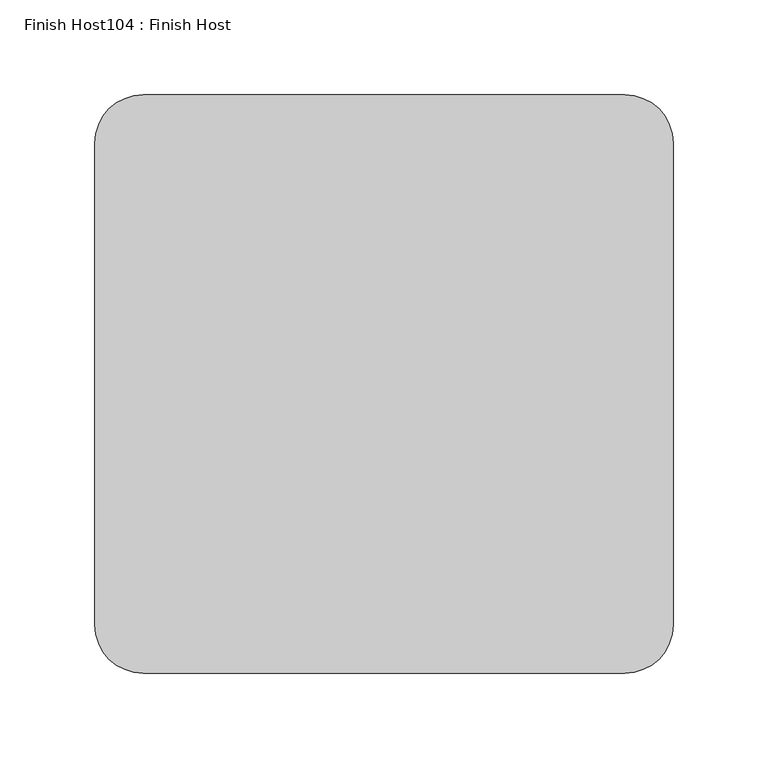
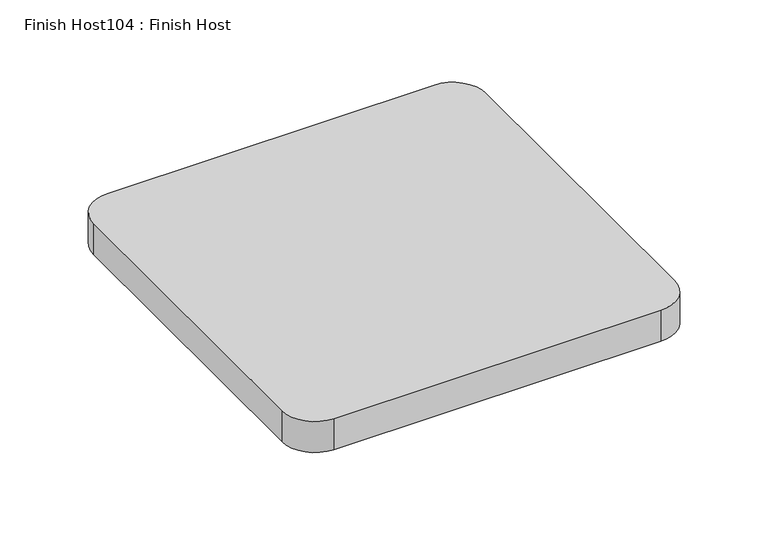
"""IFC4 building model written with IfcOpenShell, lengths in millimetres: proxy geometry, Finish Host104 : Finish Host."""

from ifc_helpers import new_model, si_unit, point, frame_2d, origin, origin_with_axes, place, context, project, spatial, polyline, circle_curve, trimmed, segment, composite_curve, outline, extrude, source, transform, mapped, element, save


def finish_host104_finish_host_b2d7b205(model_context):
    return source(origin(), model_context, "Body", "SweptSolid", [
        extrude(outline(composite_curve([segment(polyline([(701.4157184, 4229.4760864), (701.4157184, 4483.4760864)]), True, "CONTINUOUS"), segment(trimmed(circle_curve(frame_2d((726.8157184, 4483.4760864)), 25.4), [point((701.4157184, 4483.4760864))], [point((726.8157184, 4508.8760864))], False, "CARTESIAN"), True, "CONTINUOUS"), segment(polyline([(726.8157184, 4508.8760864), (980.8157184, 4508.8760864)]), True, "CONTINUOUS"), segment(trimmed(circle_curve(frame_2d((980.8157184, 4483.4760864)), 25.4), [point((980.8157184, 4508.8760864))], [point((1006.2157184, 4483.4760864))], False, "CARTESIAN"), True, "CONTINUOUS"), segment(polyline([(1006.2157184, 4483.4760864), (1006.2157184, 4229.4760864)]), True, "CONTINUOUS"), segment(trimmed(circle_curve(frame_2d((980.8157184, 4229.4760864)), 25.4), [point((1006.2157184, 4229.4760864))], [point((980.8157184, 4204.0760864))], False, "CARTESIAN"), True, "CONTINUOUS"), segment(polyline([(980.8157184, 4204.0760864), (726.8157184, 4204.0760864)]), True, "CONTINUOUS"), segment(trimmed(circle_curve(frame_2d((726.8157184, 4229.4760864)), 25.4), [point((726.8157184, 4204.0760864))], [point((701.4157184, 4229.4760864))], False, "CARTESIAN"), True, "CONTINUOUS")], self_intersect=False)), origin_with_axes(), (0.0, 0.0, 1.0), 25.4),
    ])


if __name__ == "__main__":
    model = new_model("IFC4")
    model_context = context("Model", 3, world=origin())
    ifc_project = project(units=[si_unit("LENGTHUNIT", "METRE", prefix="MILLI")], contexts=[model_context])
    site = spatial("IfcSite", under=ifc_project)
    building = spatial("IfcBuilding", under=site)
    placement = place(None, origin())
    finish_host104_finish_host_shape = finish_host104_finish_host_b2d7b205(model_context)
    element("IfcBuildingElementProxy", 1, Name="Finish Host104 : Finish Host", ObjectType="Finish Host104 : Finish Host", at=placement, inside=building, context=model_context, shape_type="MappedRepresentation", body=[
        mapped(finish_host104_finish_host_shape, transform((0.0, 0.0, 0.0), x_axis=(1.0, 0.0, 0.0), y_axis=(0.0, 1.0, 0.0), z_axis=(0.0, 0.0, 1.0))),
    ])
    save(model, "model.ifc")

# Revit data of these elements
# Type "Finish Host104 : Finish Host"
#   Countertop Material = Fabric - Teknion - P111 - Percept - Context
# Element 1 (IfcBuildingElementProxy, "Finish Host104 : Finish Host")
#   Materials on its faces: "Fabric - Teknion - P111 - Percept - Context"
# Materials
#   "Fabric - Teknion - P111 - Percept - Context": class "Generic", colour RGB 66 69 67, transparency 0, Model = "P111", Manufacturer = "Teknion Textiles", URL = "http://www.tekniontextiles.ca/", Description = "Context Percept", Cost = 0
